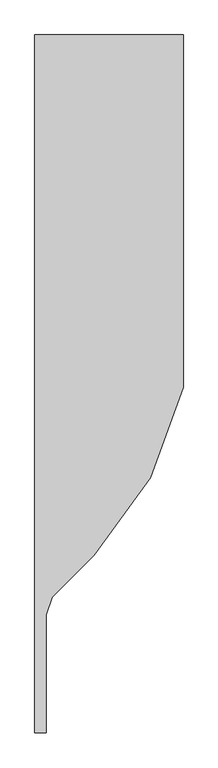
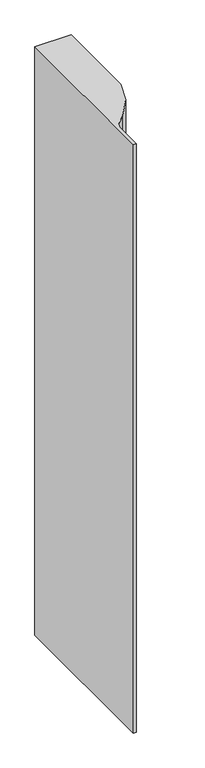
"""IFC4 building model written with IfcOpenShell, lengths in millimetres: proxy geometry, Generic Models 2:Generic Models 2:310765:Generic Models 2:310765 : Generic Models 2:Generic Models 2:310765:67 : Generic Models 2:Generic Models 2:310765:Generic Models 2:310765 : Generic Models 2:Generic Models 2:310765:300385."""

from ifc_helpers import new_model, si_unit, frame, origin, place, context, project, spatial, polyline, outline, extrude, source, transform, mapped, element, save


def generic_models_cf960079(model_context):
    return source(origin(), model_context, "Body", "SweptSolid", [
        extrude(outline(polyline([(578863.2117239, -567170.6413841), (578863.2117239, -567682.4540363), (578815.4315099, -567813.7290954), (578733.3179102, -567926.7487696), (578672.7117239, -567987.3549558), (578663.8768054, -568013.0134223), (578663.8768054, -568184.1040363), (578647.3117239, -568184.1040363), (578647.3117239, -567170.6413841), (578863.2117239, -567170.6413841)])), frame((0.0, 0.0, 4860.0679991), z_axis=(0.0, 0.0, 1.0), x_axis=(1.0, 0.0, 0.0)), (0.0, 0.0, 1.0), 3695.7),
    ])


if __name__ == "__main__":
    model = new_model("IFC4")
    model_context = context("Model", 3, world=origin())
    ifc_project = project(units=[si_unit("LENGTHUNIT", "METRE", prefix="MILLI")], contexts=[model_context])
    site = spatial("IfcSite", under=ifc_project)
    building = spatial("IfcBuilding", under=site)
    placement = place(None, origin())
    generic_models_shape = generic_models_cf960079(model_context)
    element("IfcBuildingElementProxy", 1, Name="Generic Models 2:Generic Models 2:310765:Generic Models 2:310765 : Generic Models 2:Generic Models 2:310765:67 : Generic Models 2:Generic Models 2:310765:Generic Models 2:310765 : Generic Models 2:Generic Models 2:310765:300385", ObjectType="Generic Models 2:Generic Models 2:310765:Generic Models 2:310765 : Generic Models 2:Generic Models 2:310765:67 : Generic Models 2:Generic Models 2:310765:Generic Models 2:310765 : Generic Models 2:Generic Models 2:310765:300385", at=placement, inside=building, context=model_context, shape_type="MappedRepresentation", body=[
        mapped(generic_models_shape, transform((0.0, 0.0, 0.0), x_axis=(1.0, 0.0, 0.0), y_axis=(0.0, 1.0, 0.0), z_axis=(0.0, 0.0, 1.0))),
    ])
    save(model, "model.ifc")

# Revit data of these elements
# Type "Generic Models 2:Generic Models 2:310765:Generic Models 2:310765 : Generic Models 2:Generic Models 2:310765:67 : Generic Models 2:Generic Models 2:310765:Generic Models 2:310765 : Generic Models 2:Generic Models 2:310765:300385"
#   NameOverride = "Generic Models 2:Generic Models 2:310765:Generic Models 2:310765 : Generic Models 2:Generic Models 2:310765:300385"
#   ObjectTypeOverride = "Generic Models 2:310765 : Generic Models 2:Generic Models 2:310765"
#   Reference = "Generic Models 2"
#   Tag = "300385"
# Element 1 (IfcBuildingElementProxy, "Generic Models 2:Generic Models 2:310765:Generic Models 2:310765 : Generic Models 2:Generic Models 2:310765:67 : Generic Models 2:Generic Models 2:310765:Generic Models 2:310765 : Generic Models 2:Generic Models 2:310765:300385")
#   Materials on its faces: "CLASS A FIBERGLASS INSULATION WITH DURABLE VAPOR BARRIER (WHITE) LINE"
# Materials
#   "CLASS A FIBERGLASS INSULATION WITH DURABLE VAPOR BARRIER (WHITE) LINE": class "Unassigned", colour RGB 187 139 199, transparency 0, Cost = 0
